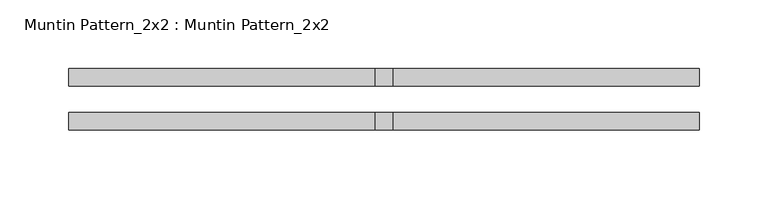
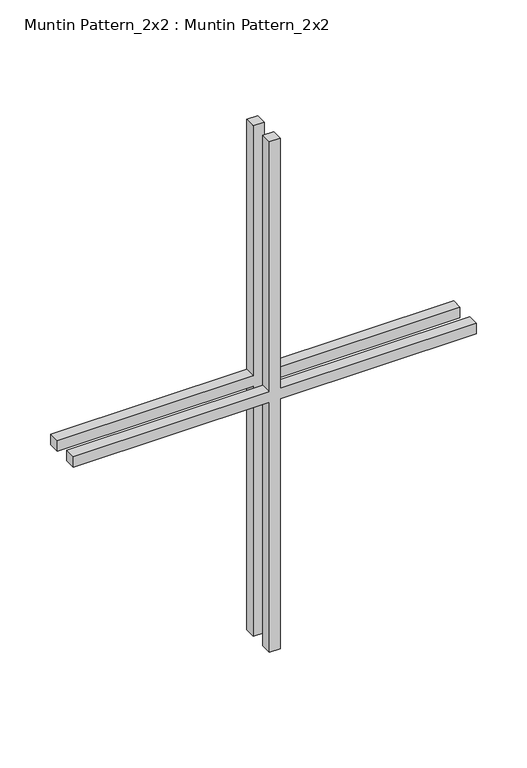
"""IFC4 building model written with IfcOpenShell, lengths in millimetres: proxy geometry, Muntin Pattern_2x2 : Muntin Pattern_2x2."""

from ifc_helpers import new_model, si_unit, frame, origin, place, context, project, spatial, polyline, outline, extrude, source, transform, mapped, element, save


def muntin_pattern_2x2_muntin_pattern_2x2_32a917e4(model_context):
    return source(origin(), model_context, "Body", "SweptSolid", [
        extrude(outline(polyline([(312.7375, -6.35), (312.7375, -228.6), (300.0375, -228.6), (300.0375, -6.35), (0.0, -6.35), (0.0, 6.35), (300.0375, 6.35), (300.0375, 228.6), (312.7375, 228.6), (312.7375, 6.35), (612.775, 6.35), (612.775, -6.35), (312.7375, -6.35)])), frame((0.0, -22.225, 0.0), z_axis=(0.0, 1.0, 0.0), x_axis=(0.0, 0.0, 1.0)), (0.0, 0.0, 1.0), 12.7),
        extrude(outline(polyline([(312.7375, -6.35), (312.7375, -228.6), (300.0375, -228.6), (300.0375, -6.35), (0.0, -6.35), (0.0, 6.35), (300.0375, 6.35), (300.0375, 228.6), (312.7375, 228.6), (312.7375, 6.35), (612.775, 6.35), (612.775, -6.35), (312.7375, -6.35)])), frame((0.0, 9.525, 0.0), z_axis=(0.0, 1.0, 0.0), x_axis=(0.0, 0.0, 1.0)), (0.0, 0.0, 1.0), 12.7),
    ])


if __name__ == "__main__":
    model = new_model("IFC4")
    model_context = context("Model", 3, world=origin())
    ifc_project = project(units=[si_unit("LENGTHUNIT", "METRE", prefix="MILLI")], contexts=[model_context])
    site = spatial("IfcSite", under=ifc_project)
    building = spatial("IfcBuilding", under=site)
    placement = place(None, origin())
    muntin_pattern_2x2_muntin_pattern_2x2_shape = muntin_pattern_2x2_muntin_pattern_2x2_32a917e4(model_context)
    element("IfcBuildingElementProxy", 1, Name="Muntin Pattern_2x2 : Muntin Pattern_2x2", ObjectType="Muntin Pattern_2x2 : Muntin Pattern_2x2", at=placement, inside=building, context=model_context, shape_type="MappedRepresentation", body=[
        mapped(muntin_pattern_2x2_muntin_pattern_2x2_shape, transform((0.0, 0.0, 0.0), x_axis=(1.0, 0.0, 0.0), y_axis=(0.0, 1.0, 0.0), z_axis=(0.0, 0.0, 1.0))),
    ])
    save(model, "model.ifc")

# Revit data of these elements
# Type "Muntin Pattern_2x2 : Muntin Pattern_2x2"
#   Width [instance default] = 4' - 0"
#   Thickness = 0' - 0 1/2"
#   Height [instance default] = 4' - 0"
#   Distance = 0' - 0 3/4"
#   Interior Material [instance default] = none
#   Exterior Material [instance default] = none
#   Default Elevation = 0
# Element 1 (IfcBuildingElementProxy, "Muntin Pattern_2x2 : Muntin Pattern_2x2")
#   Width = 1' - 6"
#   Height = 2' - 0 1/8"
#   Interior Material = Wood - Stained
#   Exterior Material = Clad - White
#   Materials on its faces: "Clad - White", "Wood - Stained"
# Materials
#   "Clad - White": class "Wood", colour RGB 245 245 243, transparency 0, Cost = 0
#   "Wood - Stained": class "Wood", colour RGB 224 178 126, transparency 0, Cost = 0
